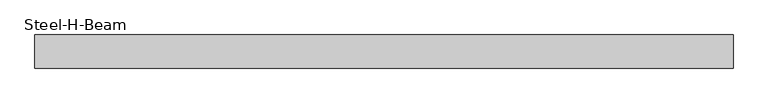
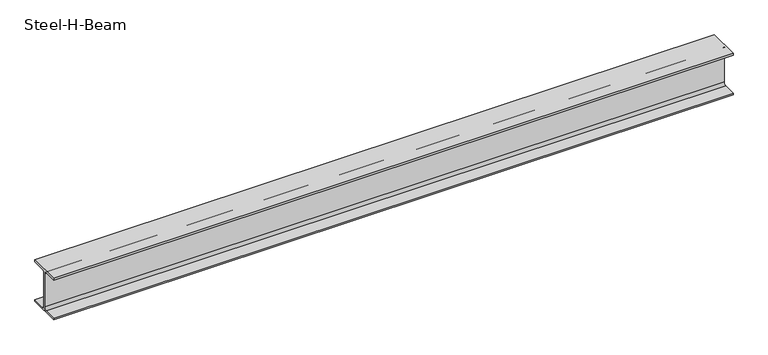
"""IFC4 building model written with IfcOpenShell, lengths in millimetres: beam geometry, Steel-H-Beam : BM121_H-340×250x9x14."""

import ifcopenshell
import ifcopenshell.guid

model = None  # the IFC model being written
_history = None  # IfcOwnerHistory: only IFC2X3 demands one
_inside = {}  # id of a spatial element -> (the spatial element, [elements in it])
_under = {}  # id of a project, library or spatial element -> (it, [spatial elements below it])
_declared = {}  # id of a project -> (the project, [libraries it declares])
_typed = {}  # id of a type object -> (the type object, [elements of that type])
_made_of = {}  # id of a material, layer set ... -> (it, [elements and type objects made of it])


def new_model(schema):
    """Start an empty IFC model of exactly this schema.

    Asked for "IFC4X3", IfcOpenShell would pick the latest addendum, in which some entities
    have other attributes; the version numbers below select the first issue.
    IFC2X3 requires an IfcOwnerHistory on every rooted entity: one is made here for all.
    """
    global model, _history
    if schema == "IFC4X3":
        model = ifcopenshell.file(schema_version=(4, 3, 0, 0))
    else:
        model = ifcopenshell.file(schema=schema)
    _inside.clear()
    _under.clear()
    _declared.clear()
    _typed.clear()
    _made_of.clear()
    _history = None
    if model.schema == "IFC2X3":
        org = make("IfcOrganization", Name="unknown")
        user = make(
            "IfcPersonAndOrganization",
            ThePerson=make("IfcPerson", FamilyName="unknown"),
            TheOrganization=org,
        )
        app = make(
            "IfcApplication",
            ApplicationDeveloper=org,
            Version="unknown",
            ApplicationFullName="unknown",
            ApplicationIdentifier="unknown",
        )
        _history = make(
            "IfcOwnerHistory",
            OwningUser=user,
            OwningApplication=app,
            ChangeAction="ADDED",
            CreationDate=0,
        )
    return model


def make(cls, **values):
    """One entity of the class cls with the attributes given. An attribute that is None is left unset."""
    return model.create_entity(
        cls, **{name: value for name, value in values.items() if value is not None}
    )


def rooted(cls, **values):
    """An entity with a GlobalId (a new one), such as an element, a storey or a relation."""
    return make(cls, GlobalId=ifcopenshell.guid.new(), OwnerHistory=_history, **values)


def si_unit(unit_type, name, prefix=None):
    """IfcSIUnit, for example si_unit("LENGTHUNIT", "METRE", prefix="MILLI")."""
    return make("IfcSIUnit", UnitType=unit_type, Prefix=prefix, Name=name)


def assignment(units):
    """IfcUnitAssignment: the units of a project."""
    return None if units is None else make("IfcUnitAssignment", Units=units)


def point(xyz):
    """IfcCartesianPoint."""
    return None if xyz is None else make("IfcCartesianPoint", Coordinates=xyz)


def direction(xyz):
    """IfcDirection."""
    return None if xyz is None else make("IfcDirection", DirectionRatios=xyz)


def frame(location, z_axis=None, x_axis=None):
    """IfcAxis2Placement3D, a coordinate frame: its origin and axes. An axis left out is left unset."""
    return make(
        "IfcAxis2Placement3D",
        Location=point(location),
        Axis=direction(z_axis),
        RefDirection=direction(x_axis),
    )


def frame_2d(location, x_axis=None):
    """IfcAxis2Placement2D, a coordinate frame in the plane: its origin and x axis."""
    return make(
        "IfcAxis2Placement2D", Location=point(location), RefDirection=direction(x_axis)
    )


def origin():
    """The frame at (0, 0, 0) with its axes left unset."""
    return frame((0.0, 0.0, 0.0))


def place(relative_to, where):
    """IfcLocalPlacement: puts the frame where relative to a parent placement (None: the world)."""
    return make(
        "IfcLocalPlacement", PlacementRelTo=relative_to, RelativePlacement=where
    )


def context(
    kind, dimensions, precision=None, world=None, true_north=None, identifier=None
):
    """IfcGeometricRepresentationContext, for example the 3D "Model" context."""
    return make(
        "IfcGeometricRepresentationContext",
        ContextIdentifier=identifier,
        ContextType=kind,
        CoordinateSpaceDimension=dimensions,
        Precision=precision,
        WorldCoordinateSystem=world,
        TrueNorth=true_north,
    )


def project(units=None, contexts=None):
    """IfcProject with its units and contexts."""
    return rooted(
        "IfcProject",
        Name="project",
        RepresentationContexts=contexts,
        UnitsInContext=assignment(units),
    )


def spatial(cls, under=None, at=None, **own):
    """A site, building, storey or space (cls), placed at a placement, below another one or the project."""
    s = rooted(cls, ObjectPlacement=at, **own)
    if under is not None:
        _under.setdefault(under.id(), (under, []))[1].append(s)
    return s


def polyline(points):
    """IfcPolyline through the points."""
    return make("IfcPolyline", Points=[point(p) for p in points])


def circle_curve(where, radius):
    """IfcCircle in the frame where."""
    return make("IfcCircle", Position=where, Radius=radius)


def trimmed(basis, trim1, trim2, sense, master):
    """IfcTrimmedCurve: the piece of a basis curve between two trims."""
    return make(
        "IfcTrimmedCurve",
        BasisCurve=basis,
        Trim1=trim1,
        Trim2=trim2,
        SenseAgreement=sense,
        MasterRepresentation=master,
    )


def segment(curve, same_sense, transition):
    """IfcCompositeCurveSegment."""
    return make(
        "IfcCompositeCurveSegment",
        Transition=transition,
        SameSense=same_sense,
        ParentCurve=curve,
    )


def composite_curve(segments, self_intersect=None):
    """IfcCompositeCurve: segments joined end to end."""
    return make("IfcCompositeCurve", Segments=segments, SelfIntersect=self_intersect)


def outline(outer, holes=None, kind="AREA"):
    """IfcArbitraryClosedProfileDef: a profile drawn as a closed curve; with holes, ...WithVoids."""
    if holes is None:
        return make("IfcArbitraryClosedProfileDef", ProfileType=kind, OuterCurve=outer)
    return make(
        "IfcArbitraryProfileDefWithVoids",
        ProfileType=kind,
        OuterCurve=outer,
        InnerCurves=holes,
    )


def extrude(swept, where, along, depth):
    """IfcExtrudedAreaSolid: the profile swept, set in the frame where, extruded along a direction by depth."""
    return make(
        "IfcExtrudedAreaSolid",
        SweptArea=swept,
        Position=where,
        ExtrudedDirection=direction(along),
        Depth=depth,
    )


def shape(context_of_items, identifier, shape_type, items):
    """IfcShapeRepresentation: the items that make up one representation, for example the "Body"."""
    return make(
        "IfcShapeRepresentation",
        ContextOfItems=context_of_items,
        RepresentationIdentifier=identifier,
        RepresentationType=shape_type,
        Items=items,
    )


def source(mapping_origin, context_of_items, identifier, shape_type, items):
    """IfcRepresentationMap: a shape defined once, which mapped items show again and again."""
    return make(
        "IfcRepresentationMap",
        MappingOrigin=mapping_origin,
        MappedRepresentation=shape(context_of_items, identifier, shape_type, items),
    )


def transform(
    local_origin,
    x_axis=None,
    y_axis=None,
    z_axis=None,
    scale=None,
    scale2=None,
    scale3=None,
    uniform=True,
):
    """IfcCartesianTransformationOperator3D, or its non-uniform kind. x_axis, y_axis, z_axis: its Axis1, 2, 3."""
    if uniform:
        return make(
            "IfcCartesianTransformationOperator3D",
            Axis1=direction(x_axis),
            Axis2=direction(y_axis),
            LocalOrigin=point(local_origin),
            Scale=scale,
            Axis3=direction(z_axis),
        )
    return make(
        "IfcCartesianTransformationOperator3DnonUniform",
        Axis1=direction(x_axis),
        Axis2=direction(y_axis),
        LocalOrigin=point(local_origin),
        Scale=scale,
        Axis3=direction(z_axis),
        Scale2=scale2,
        Scale3=scale3,
    )


def mapped(mapping_source, mapping_target):
    """IfcMappedItem: shows the shape of a source again, moved by a transform."""
    return make(
        "IfcMappedItem", MappingSource=mapping_source, MappingTarget=mapping_target
    )


def made_of(thing, what):
    """Note that an element or type object is made of a material, layer set ...; save() writes the relation."""
    if what is not None:
        _made_of.setdefault(what.id(), (what, []))[1].append(thing)
    return thing


def element(
    cls,
    number,
    at=None,
    inside=None,
    cuts=None,
    type_object=None,
    material=None,
    context=None,
    identifier="Body",
    shape_type=None,
    held_by="IfcProductDefinitionShape",
    body=None,
    shapes=None,
    **own,
):
    """One element of the class cls, such as IfcWall. Its Tag is "e" and its number.

    at: its placement. inside: the storey or other place that contains it. cuts: it is an
    opening in that element (IfcRelVoidsElement). A single representation is given by context,
    identifier, shape_type and body (its items); several are given by shapes. held_by: the class
    of the entity that holds the representations. save() writes the other relations.
    """
    e = rooted(cls, Tag="e%d" % number, ObjectPlacement=at, **own)
    if body is not None:
        shapes = [shape(context, identifier, shape_type, body)]
    if shapes is not None:
        e.Representation = make(held_by, Representations=shapes)
    if inside is not None:
        _inside.setdefault(inside.id(), (inside, []))[1].append(e)
    if cuts is not None:
        rooted(
            "IfcRelVoidsElement", RelatingBuildingElement=cuts, RelatedOpeningElement=e
        )
    if type_object is not None:
        _typed.setdefault(type_object.id(), (type_object, []))[1].append(e)
    return made_of(e, material)


def aggregate(whole, parts):
    """IfcRelAggregates: a whole, such as a stair, and the parts it consists of."""
    return rooted("IfcRelAggregates", RelatingObject=whole, RelatedObjects=parts)


def save(model, path):
    """Write the relations noted so far, then the file.

    IfcRelAggregates (storeys below a building ...), IfcRelContainedInSpatialStructure (elements
    in a storey), IfcRelDefinesByType, IfcRelAssociatesMaterial and IfcRelDeclares: one each for
    every whole, place, type object, material and project.
    """
    for whole, parts in _under.values():
        aggregate(whole, parts)
    for where, things in _inside.values():
        rooted(
            "IfcRelContainedInSpatialStructure",
            RelatedElements=things,
            RelatingStructure=where,
        )
    for kind, things in _typed.values():
        rooted("IfcRelDefinesByType", RelatedObjects=things, RelatingType=kind)
    for what, things in _made_of.values():
        rooted("IfcRelAssociatesMaterial", RelatedObjects=things, RelatingMaterial=what)
    for by, libraries in _declared.values():
        rooted("IfcRelDeclares", RelatingContext=by, RelatedDefinitions=libraries)
    model.write(path)


def steel_h_beam_04323a77(model_context):
    return source(origin(), model_context, "Body", "SweptSolid", [
        extrude(outline(composite_curve([segment(polyline([(125.0, -156.0), (125.0, -170.0), (-125.0, -170.0), (-125.0, -156.0), (-24.5, -156.0)]), True, "CONTINUOUS"), segment(trimmed(circle_curve(frame_2d((-24.5, -136.0)), 20.0), [point((-24.5, -156.0))], [point((-4.5, -136.0))], True, "CARTESIAN"), True, "CONTINUOUS"), segment(polyline([(-4.5, -136.0), (-4.5, 136.0)]), True, "CONTINUOUS"), segment(trimmed(circle_curve(frame_2d((-24.5, 136.0)), 20.0), [point((-4.5, 136.0))], [point((-24.5, 156.0))], True, "CARTESIAN"), True, "CONTINUOUS"), segment(polyline([(-24.5, 156.0), (-125.0, 156.0), (-125.0, 170.0), (125.0, 170.0), (125.0, 156.0), (24.5, 156.0)]), True, "CONTINUOUS"), segment(trimmed(circle_curve(frame_2d((24.5, 136.0)), 20.0), [point((24.5, 156.0))], [point((4.5, 136.0))], True, "CARTESIAN"), True, "CONTINUOUS"), segment(polyline([(4.5, 136.0), (4.5, -136.0)]), True, "CONTINUOUS"), segment(trimmed(circle_curve(frame_2d((24.5, -136.0)), 20.0), [point((4.5, -136.0))], [point((24.5, -156.0))], True, "CARTESIAN"), True, "CONTINUOUS"), segment(polyline([(24.5, -156.0), (125.0, -156.0)]), True, "CONTINUOUS")], self_intersect=False)), frame((-2524.0357919, 0.0, 0.0), z_axis=(1.0, 0.0, 0.0), x_axis=(0.0, 1.0, 0.0)), (0.0, 0.0, 1.0), 5262.1606688),
    ])


if __name__ == "__main__":
    model = new_model("IFC4")
    model_context = context("Model", 3, world=origin())
    ifc_project = project(units=[si_unit("LENGTHUNIT", "METRE", prefix="MILLI")], contexts=[model_context])
    site = spatial("IfcSite", under=ifc_project)
    building = spatial("IfcBuilding", under=site)
    placement = place(None, origin())
    steel_h_beam_shape = steel_h_beam_04323a77(model_context)
    element("IfcBeam", 1, ObjectType="Steel-H-Beam : BM121_H-340×250x9x14", at=placement, inside=building, context=model_context, shape_type="MappedRepresentation", body=[
        mapped(steel_h_beam_shape, transform((0.0, 0.0, 0.0), x_axis=(1.0, 0.0, 0.0), y_axis=(0.0, 1.0, 0.0), z_axis=(0.0, 0.0, 1.0))),
    ])
    save(model, "model.ifc")

# Revit data of these elements
# Type "Steel-H-Beam : BM121_H-340×250x9x14"
#   Surface Area = 1.62766 m²/m
#   Section Area = 101.514 cm²
#   Mass per Unit Length = 79.6882 kg/m
#   Length [instance default] = 3000 mm
#   B = 250 mm
#   H = 340 mm
#   r = 20 mm
#   tw = 9 mm
#   tf = 14 mm
#   hec_material4 [instance default] = none
#   hec_material3 [instance default] = none
#   hec_material2 [instance default] = none
#   hec_material1 [instance default] = none
#   Structural Material [instance default] = Steel, 45-345
#   Assembly Code = ""
# Element 1 (IfcBeam, "Steel-H-Beam : BM121_H-340×250x9x14")
#   hec_material4 = S01AA010-00002_Main Steel Structure Fabrication Work_Shelter/Building_Steel Painting/Coating_for Fireproofed Steel Surface, Surface Preparation & Primer Coat
#   hec_material3 = F01AC000-00002_Building/Shelter Fire Proofing Work_Intumescent Coating Type_1 hr. rating (UL 1709))
#   hec_material2 = S01AA010-00002_Main Steel Structure Fabrication Work_Shelter/Building_Steel Painting/Coating_for Fireproofed Steel Surface, Surface Preparation & Primer Coat
#   hec_material1 = S03AA028-00001_Main Steel Structure Erection Work_Shelter/Building_Medium Steel
#   Structural Material = S01AA002-00001_Main Steel Structure Fabrication Work_Shelter/Building_Medium Steel - Standard
#   Materials on its faces: "S01AA002-00001_Main Steel Structure Fabrication Work_Shelter/Building_Medium Steel - Standard"
# Materials
#   "Steel, 45-345": class "Metal", colour RGB 189 187 185, transparency 0, Description = "Steel 345 MPa", Cost = 0
#   "S01AA002-00001_Main Steel Structure Fabrication Work_Shelter/Building_Medium Steel - Standard": class "Metal", colour RGB 120 120 120, transparency 0, Comments = "(90KG/M>Weight≥30KG/M)", Description = "Structural steel 50ksi", W00) Work Master Code = "S01AA002-0001", W01) Work Master_Lv1 = "Main Steel Structure Fabrication Work", W02) Work Master_Lv2 = "Shelter/Building", W03) Work Master_Spec.1 = "Medium Steel - Standard (90KG/M>Weight≥30KG/M)", Cost = 0
#   "S01AA010-00002_Main Steel Structure Fabrication Work_Shelter/Building_Steel Painting/Coating_for Fireproofed Steel Surface, Surface Preparation & Primer Coat": class "Metal", colour RGB 120 120 120, transparency 0, Description = "Paint finished steel", W00) Work Master Code = "SS01AA010-00002", W01) Work Master_Lv1 = "Main Steel Structure Fabrication Work", W02) Work Master_Lv2 = "Shelter/Building", W03) Work Master_Spec.1 = "Steel Painting/Coating", W04) Work Master_Spec.2 = "for Fireproofed Steel Surface, Surface Preparation & Primer Coat", Cost = 0
#   "F01AC000-00002_Building/Shelter Fire Proofing Work_Intumescent Coating Type_1 hr. rating (UL 1709))": class "Metal", colour RGB 255 128 128, transparency 0, Description = "Paint finished steel", W00) Work Master Code = "F01AC000-00002", W01) Work Master_Lv1 = "Building/Shelter Fire Proofing Work", W02) Work Master_Lv2 = "Intumescent Coating Type", W03) Work Master_Spec.1 = "1 hr. rating (UL 1709)", Cost = 0
#   "S03AA028-00001_Main Steel Structure Erection Work_Shelter/Building_Medium Steel": class "Metal", colour RGB 120 120 120, transparency 0, Comments = "(90KG/M>Weight≥30KG/M)", Description = "Structural steel 50ksi", W00) Work Master Code = "S03AA028-0001", W01) Work Master_Lv1 = "Main Steel Structure Erection Work", W02) Work Master_Lv2 = "Shelter/Building", W03) Work Master_Spec.1 = "Medium Steel (90KG/M>Weight≥30KG/M)", Cost = 0
